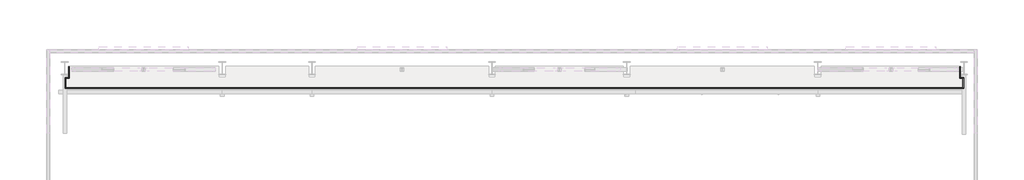
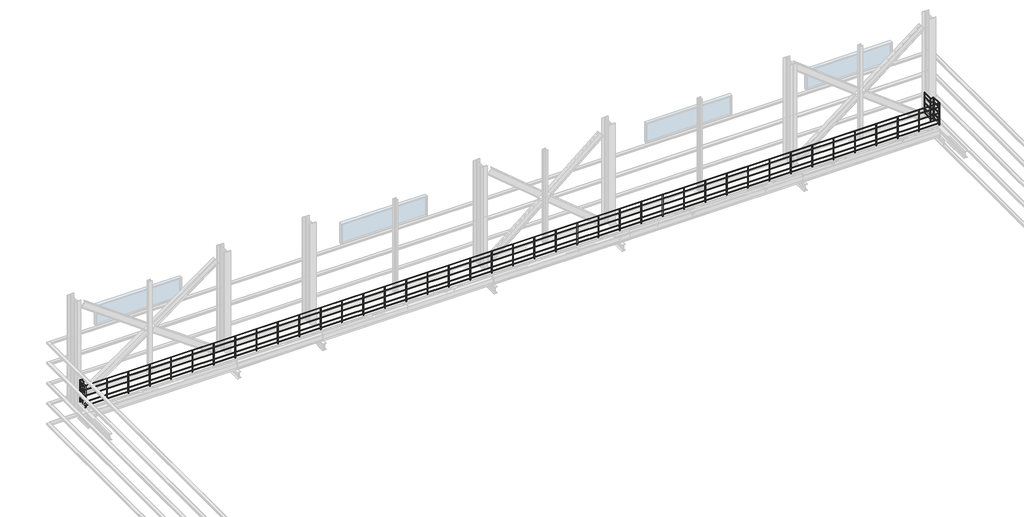
# One storey, part 4 of 4: 1 railing.
"""IFC4 building model written with IfcOpenShell, lengths in millimetres."""

import ifcopenshell
import ifcopenshell.guid

model = None  # the IFC model being written
_history = None  # IfcOwnerHistory: only IFC2X3 demands one
_inside = {}  # id of a spatial element -> (the spatial element, [elements in it])
_under = {}  # id of a project, library or spatial element -> (it, [spatial elements below it])
_declared = {}  # id of a project -> (the project, [libraries it declares])
_typed = {}  # id of a type object -> (the type object, [elements of that type])
_made_of = {}  # id of a material, layer set ... -> (it, [elements and type objects made of it])


def new_model(schema):
    """Start an empty IFC model of exactly this schema.

    Asked for "IFC4X3", IfcOpenShell would pick the latest addendum, in which some entities
    have other attributes; the version numbers below select the first issue.
    IFC2X3 requires an IfcOwnerHistory on every rooted entity: one is made here for all.
    """
    global model, _history
    if schema == "IFC4X3":
        model = ifcopenshell.file(schema_version=(4, 3, 0, 0))
    else:
        model = ifcopenshell.file(schema=schema)
    _inside.clear()
    _under.clear()
    _declared.clear()
    _typed.clear()
    _made_of.clear()
    _history = None
    if model.schema == "IFC2X3":
        org = make("IfcOrganization", Name="unknown")
        user = make(
            "IfcPersonAndOrganization",
            ThePerson=make("IfcPerson", FamilyName="unknown"),
            TheOrganization=org,
        )
        app = make(
            "IfcApplication",
            ApplicationDeveloper=org,
            Version="unknown",
            ApplicationFullName="unknown",
            ApplicationIdentifier="unknown",
        )
        _history = make(
            "IfcOwnerHistory",
            OwningUser=user,
            OwningApplication=app,
            ChangeAction="ADDED",
            CreationDate=0,
        )
    return model


def make(cls, **values):
    """One entity of the class cls with the attributes given. An attribute that is None is left unset."""
    return model.create_entity(
        cls, **{name: value for name, value in values.items() if value is not None}
    )


def rooted(cls, **values):
    """An entity with a GlobalId (a new one), such as an element, a storey or a relation."""
    return make(cls, GlobalId=ifcopenshell.guid.new(), OwnerHistory=_history, **values)


def si_unit(unit_type, name, prefix=None):
    """IfcSIUnit, for example si_unit("LENGTHUNIT", "METRE", prefix="MILLI")."""
    return make("IfcSIUnit", UnitType=unit_type, Prefix=prefix, Name=name)


def assignment(units):
    """IfcUnitAssignment: the units of a project."""
    return None if units is None else make("IfcUnitAssignment", Units=units)


def point(xyz):
    """IfcCartesianPoint."""
    return None if xyz is None else make("IfcCartesianPoint", Coordinates=xyz)


def direction(xyz):
    """IfcDirection."""
    return None if xyz is None else make("IfcDirection", DirectionRatios=xyz)


def frame(location, z_axis=None, x_axis=None):
    """IfcAxis2Placement3D, a coordinate frame: its origin and axes. An axis left out is left unset."""
    return make(
        "IfcAxis2Placement3D",
        Location=point(location),
        Axis=direction(z_axis),
        RefDirection=direction(x_axis),
    )


def origin():
    """The frame at (0, 0, 0) with its axes left unset."""
    return frame((0.0, 0.0, 0.0))


def place(relative_to, where):
    """IfcLocalPlacement: puts the frame where relative to a parent placement (None: the world)."""
    return make(
        "IfcLocalPlacement", PlacementRelTo=relative_to, RelativePlacement=where
    )


def context(
    kind, dimensions, precision=None, world=None, true_north=None, identifier=None
):
    """IfcGeometricRepresentationContext, for example the 3D "Model" context."""
    return make(
        "IfcGeometricRepresentationContext",
        ContextIdentifier=identifier,
        ContextType=kind,
        CoordinateSpaceDimension=dimensions,
        Precision=precision,
        WorldCoordinateSystem=world,
        TrueNorth=true_north,
    )


def project(units=None, contexts=None):
    """IfcProject with its units and contexts."""
    return rooted(
        "IfcProject",
        Name="project",
        RepresentationContexts=contexts,
        UnitsInContext=assignment(units),
    )


def spatial(cls, under=None, at=None, **own):
    """A site, building, storey or space (cls), placed at a placement, below another one or the project."""
    s = rooted(cls, ObjectPlacement=at, **own)
    if under is not None:
        _under.setdefault(under.id(), (under, []))[1].append(s)
    return s


def polyline(points):
    """IfcPolyline through the points."""
    return make("IfcPolyline", Points=[point(p) for p in points])


def circle_curve(where, radius):
    """IfcCircle in the frame where."""
    return make("IfcCircle", Position=where, Radius=radius)


def ellipse_curve(where, semi_axis1, semi_axis2):
    """IfcEllipse in the frame where."""
    return make(
        "IfcEllipse", Position=where, SemiAxis1=semi_axis1, SemiAxis2=semi_axis2
    )


def outline(outer, holes=None, kind="AREA"):
    """IfcArbitraryClosedProfileDef: a profile drawn as a closed curve; with holes, ...WithVoids."""
    if holes is None:
        return make("IfcArbitraryClosedProfileDef", ProfileType=kind, OuterCurve=outer)
    return make(
        "IfcArbitraryProfileDefWithVoids",
        ProfileType=kind,
        OuterCurve=outer,
        InnerCurves=holes,
    )


def extrude(swept, where, along, depth):
    """IfcExtrudedAreaSolid: the profile swept, set in the frame where, extruded along a direction by depth."""
    return make(
        "IfcExtrudedAreaSolid",
        SweptArea=swept,
        Position=where,
        ExtrudedDirection=direction(along),
        Depth=depth,
    )


def shape(context_of_items, identifier, shape_type, items):
    """IfcShapeRepresentation: the items that make up one representation, for example the "Body"."""
    return make(
        "IfcShapeRepresentation",
        ContextOfItems=context_of_items,
        RepresentationIdentifier=identifier,
        RepresentationType=shape_type,
        Items=items,
    )


def made_of(thing, what):
    """Note that an element or type object is made of a material, layer set ...; save() writes the relation."""
    if what is not None:
        _made_of.setdefault(what.id(), (what, []))[1].append(thing)
    return thing


def element(
    cls,
    number,
    at=None,
    inside=None,
    cuts=None,
    type_object=None,
    material=None,
    context=None,
    identifier="Body",
    shape_type=None,
    held_by="IfcProductDefinitionShape",
    body=None,
    shapes=None,
    **own,
):
    """One element of the class cls, such as IfcWall. Its Tag is "e" and its number.

    at: its placement. inside: the storey or other place that contains it. cuts: it is an
    opening in that element (IfcRelVoidsElement). A single representation is given by context,
    identifier, shape_type and body (its items); several are given by shapes. held_by: the class
    of the entity that holds the representations. save() writes the other relations.
    """
    e = rooted(cls, Tag="e%d" % number, ObjectPlacement=at, **own)
    if body is not None:
        shapes = [shape(context, identifier, shape_type, body)]
    if shapes is not None:
        e.Representation = make(held_by, Representations=shapes)
    if inside is not None:
        _inside.setdefault(inside.id(), (inside, []))[1].append(e)
    if cuts is not None:
        rooted(
            "IfcRelVoidsElement", RelatingBuildingElement=cuts, RelatedOpeningElement=e
        )
    if type_object is not None:
        _typed.setdefault(type_object.id(), (type_object, []))[1].append(e)
    return made_of(e, material)


def aggregate(whole, parts):
    """IfcRelAggregates: a whole, such as a stair, and the parts it consists of."""
    return rooted("IfcRelAggregates", RelatingObject=whole, RelatedObjects=parts)


def save(model, path):
    """Write the relations noted so far, then the file.

    IfcRelAggregates (storeys below a building ...), IfcRelContainedInSpatialStructure (elements
    in a storey), IfcRelDefinesByType, IfcRelAssociatesMaterial and IfcRelDeclares: one each for
    every whole, place, type object, material and project.
    """
    for whole, parts in _under.values():
        aggregate(whole, parts)
    for where, things in _inside.values():
        rooted(
            "IfcRelContainedInSpatialStructure",
            RelatedElements=things,
            RelatingStructure=where,
        )
    for kind, things in _typed.values():
        rooted("IfcRelDefinesByType", RelatedObjects=things, RelatingType=kind)
    for what, things in _made_of.values():
        rooted("IfcRelAssociatesMaterial", RelatedObjects=things, RelatingMaterial=what)
    for by, libraries in _declared.values():
        rooted("IfcRelDeclares", RelatingContext=by, RelatedDefinitions=libraries)
    model.write(path)


def plane_surface(at):
    """IfcPlane: the flat surface through the origin of the frame at, square to its z axis."""
    return make("IfcPlane", Position=at)


def cylinder_surface(at, radius):
    """IfcCylindricalSurface: all points at the distance radius from the z axis of the frame at."""
    return make("IfcCylindricalSurface", Position=at, Radius=radius)


def advanced_brep(points, edges, surfaces, faces):
    """IfcAdvancedBrep: a solid bounded by faces that lie on surfaces and meet in shared edges.

    An edge is (start, end): straight between two places in points (the first is 0);
    or (start, end, curve); or (start, end, curve, False) where it runs against its curve.
    A face is (place in surfaces, loops), or (place, loops, False) where it looks against
    its surface's normal. A loop lists edges by number (the first is 1), with a minus sign
    where the edge is run from its end to its start. The first loop is the outer one.
    """
    corners = [point(p) for p in points]
    vertices = [make("IfcVertexPoint", VertexGeometry=c) for c in corners]
    made = []
    for start, end, *more in edges:
        made.append(
            make(
                "IfcEdgeCurve",
                EdgeStart=vertices[start],
                EdgeEnd=vertices[end],
                EdgeGeometry=more[0] if more else make("IfcPolyline", Points=[corners[start], corners[end]]),
                SameSense=more[1] if len(more) > 1 else True,
            )
        )
    hull = []
    for where, loops, *sense in faces:
        bounds = []
        for j, loop in enumerate(loops):
            ring = [make("IfcOrientedEdge", EdgeElement=made[abs(k) - 1], Orientation=k > 0) for k in loop]
            bounds.append(
                make(
                    "IfcFaceOuterBound" if j == 0 else "IfcFaceBound",
                    Bound=make("IfcEdgeLoop", EdgeList=ring),
                    Orientation=True,
                )
            )
        hull.append(make("IfcAdvancedFace", Bounds=bounds, FaceSurface=surfaces[where], SameSense=sense[0] if sense else True))
    return make("IfcAdvancedBrep", Outer=make("IfcClosedShell", CfsFaces=hull))


model = new_model("IFC4")

# Units and contexts
model_context = context("Model", 3, world=origin())
ifc_project = project(units=[si_unit("LENGTHUNIT", "METRE", prefix="MILLI")], contexts=[model_context])

# Site, building, storey
site = spatial("IfcSite", under=ifc_project)
building = spatial("IfcBuilding", under=site)
storey = spatial("IfcBuildingStorey", under=building, Name="T.O.CRANE GIR.", Elevation=12299.9720055)

# Railing
placement = place(None, origin())
element("IfcRailing", 1, ObjectType="RA101_1100mm", at=placement, inside=storey, context=model_context, shape_type="SolidModel", body=[
    advanced_brep(
    [(165.0, 39119.5208589, 13466.9720055), (195.0, 39119.5208589, 13466.9720055), (165.0, 38634.5208589, 13466.9720055), (195.0, 38604.5208589, 13466.9720055), (15.0, 38634.5208589, 13466.9720055), (45.0, 38604.5208589, 13466.9720055), (15.0, 38164.5208589, 13466.9720055), (45.0, 38194.5208589, 13466.9720055), (39985.0, 38164.5208589, 13466.9720055), (39955.0, 38194.5208589, 13466.9720055), (39985.0, 38634.5208589, 13466.9720055), (39955.0, 38604.5208589, 13466.9720055), (39835.0, 38634.5208589, 13466.9720055), (39805.0, 38604.5208589, 13466.9720055), (39835.0, 39119.5208589, 13466.9720055), (39805.0, 39119.5208589, 13466.9720055)],
    [
        (0, 1, circle_curve(frame((180.0, 39119.5208589, 13466.9720055), z_axis=(0.0, 1.0, 0.0), x_axis=(1.0, 0.0, 0.0)), 15.0)),
        (1, 0, circle_curve(frame((180.0, 39119.5208589, 13466.9720055), z_axis=(0.0, 1.0, 0.0), x_axis=(1.0, 0.0, 0.0)), 15.0)),
        (0, 2),
        (2, 3, ellipse_curve(frame((180.0, 38619.5208589, 13466.9720055), z_axis=(0.707106781186548, 0.7071067811865469, 0.0), x_axis=(-0.7071067811865468, 0.7071067811865482, 0.0)), 21.2132034, 15.0)),
        (3, 1),
        (3, 2, ellipse_curve(frame((180.0, 38619.5208589, 13466.9720055), z_axis=(0.707106781186548, 0.7071067811865469, 0.0), x_axis=(-0.7071067811865468, 0.7071067811865482, 0.0)), 21.2132034, 15.0)),
        (2, 4),
        (4, 5, ellipse_curve(frame((30.0, 38619.5208589, 13466.9720055), z_axis=(0.707106781186548, 0.7071067811865469, 0.0), x_axis=(0.7071067811865472, -0.7071067811865479, 0.0)), 21.2132034, 15.0)),
        (5, 3),
        (5, 4, ellipse_curve(frame((30.0, 38619.5208589, 13466.9720055), z_axis=(0.707106781186548, 0.7071067811865469, 0.0), x_axis=(0.7071067811865472, -0.7071067811865479, 0.0)), 21.2132034, 15.0)),
        (4, 6),
        (6, 7, ellipse_curve(frame((30.0, 38179.5208589, 13466.9720055), z_axis=(-0.7071067811865459, 0.7071067811865491, 0.0), x_axis=(0.7071067811865491, 0.7071067811865458, 0.0)), 21.2132034, 15.0)),
        (7, 5),
        (7, 6, ellipse_curve(frame((30.0, 38179.5208589, 13466.9720055), z_axis=(-0.7071067811865459, 0.7071067811865491, 0.0), x_axis=(0.7071067811865491, 0.7071067811865458, 0.0)), 21.2132034, 15.0)),
        (6, 8),
        (8, 9, ellipse_curve(frame((39970.0, 38179.5208589, 13466.9720055), z_axis=(-0.7071067811865486, -0.7071067811865465, 0.0), x_axis=(-0.7071067811865465, 0.7071067811865486, 0.0)), 21.2132034, 15.0)),
        (9, 7),
        (9, 8, ellipse_curve(frame((39970.0, 38179.5208589, 13466.9720055), z_axis=(-0.7071067811865486, -0.7071067811865465, 0.0), x_axis=(-0.7071067811865465, 0.7071067811865486, 0.0)), 21.2132034, 15.0)),
        (8, 10),
        (10, 11, ellipse_curve(frame((39970.0, 38619.5208589, 13466.9720055), z_axis=(0.7071067811865476, -0.7071067811865474, 0.0), x_axis=(-0.7071067811865472, -0.7071067811865478, 0.0)), 21.2132034, 15.0)),
        (11, 9),
        (11, 10, ellipse_curve(frame((39970.0, 38619.5208589, 13466.9720055), z_axis=(0.7071067811865476, -0.7071067811865474, 0.0), x_axis=(-0.7071067811865472, -0.7071067811865478, 0.0)), 21.2132034, 15.0)),
        (10, 12),
        (12, 13, ellipse_curve(frame((39820.0, 38619.5208589, 13466.9720055), z_axis=(0.7071067811865476, -0.7071067811865474, 0.0), x_axis=(0.7071067811865475, 0.7071067811865475, 0.0)), 21.2132034, 15.0)),
        (13, 11),
        (13, 12, ellipse_curve(frame((39820.0, 38619.5208589, 13466.9720055), z_axis=(0.7071067811865476, -0.7071067811865474, 0.0), x_axis=(0.7071067811865475, 0.7071067811865475, 0.0)), 21.2132034, 15.0)),
        (14, 15, circle_curve(frame((39820.0, 39119.5208589, 13466.9720055), z_axis=(0.0, 1.0, 0.0), x_axis=(-1.0, 0.0, 0.0)), 15.0)),
        (15, 14, circle_curve(frame((39820.0, 39119.5208589, 13466.9720055), z_axis=(0.0, 1.0, 0.0), x_axis=(-1.0, 0.0, 0.0)), 15.0)),
        (12, 14),
        (15, 13),
    ],
    [
        plane_surface(frame((180.0, 39119.5208589, 13481.9720055), z_axis=(0.0, 1.0, 0.0), x_axis=(0.0, 0.0, -1.0))),
        cylinder_surface(frame((180.0, 39119.5208589, 13466.9720055), z_axis=(0.0, 1.0, 0.0), x_axis=(1.0, 0.0, 0.0)), 15.0),
        cylinder_surface(frame((180.0, 38619.5208589, 13466.9720055), z_axis=(1.0, 0.0, 0.0), x_axis=(0.0, -1.0, 0.0)), 15.0),
        cylinder_surface(frame((30.0, 38619.5208589, 13466.9720055), z_axis=(0.0, 1.0, 0.0), x_axis=(1.0, 0.0, 0.0)), 15.0),
        cylinder_surface(frame((30.0, 38179.5208589, 13466.9720055), z_axis=(-1.0, 0.0, 0.0), x_axis=(0.0, 1.0, 0.0)), 15.0),
        cylinder_surface(frame((39970.0, 38179.5208589, 13466.9720055), z_axis=(0.0, -1.0, 0.0), x_axis=(-1.0, 0.0, 0.0)), 15.0),
        cylinder_surface(frame((39970.0, 38619.5208589, 13466.9720055), z_axis=(1.0, 0.0, 0.0), x_axis=(0.0, -1.0, 0.0)), 15.0),
        plane_surface(frame((39820.0, 39119.5208589, 13481.9720055), z_axis=(0.0, 1.0, 0.0), x_axis=(0.0, 0.0, 1.0))),
        cylinder_surface(frame((39820.0, 38619.5208589, 13466.9720055), z_axis=(0.0, -1.0, 0.0), x_axis=(-1.0, 0.0, 0.0)), 15.0),
    ],
    [
        (0, [[1, 2]]),
        (1, [[-1, 3, 4, 5]]),
        (1, [[-2, -5, 6, -3]]),
        (2, [[-4, 7, 8, 9]]),
        (2, [[-6, -9, 10, -7]]),
        (3, [[-8, 11, 12, 13]]),
        (3, [[-10, -13, 14, -11]]),
        (4, [[-12, 15, 16, 17]]),
        (4, [[-14, -17, 18, -15]]),
        (5, [[-16, 19, 20, 21]]),
        (5, [[-18, -21, 22, -19]]),
        (6, [[-20, 23, 24, 25]]),
        (6, [[-22, -25, 26, -23]]),
        (7, [[27, 28]]),
        (8, [[-24, 29, -28, 30]]),
        (8, [[-26, -30, -27, -29]]),
    ],
),
    advanced_brep(
    [(15.0, 38634.5208589, 13266.9720055), (45.0, 38604.5208589, 13266.9720055), (45.0, 38194.5208589, 13266.9720055), (15.0, 38164.5208589, 13266.9720055), (39955.0, 38194.5208589, 13266.9720055), (39985.0, 38164.5208589, 13266.9720055), (39955.0, 38604.5208589, 13266.9720055), (39985.0, 38634.5208589, 13266.9720055), (39805.0, 38604.5208589, 13266.9720055), (39835.0, 38634.5208589, 13266.9720055), (39805.0, 39119.5208589, 13266.9720055), (39835.0, 39119.5208589, 13266.9720055), (195.0, 39119.5208589, 13266.9720055), (165.0, 39119.5208589, 13266.9720055), (195.0, 38604.5208589, 13266.9720055), (165.0, 38634.5208589, 13266.9720055)],
    [
        (0, 1, ellipse_curve(frame((30.0, 38619.5208589, 13266.9720055), z_axis=(-0.707106781186548, -0.7071067811865469, 0.0), x_axis=(-0.7071067811865467, 0.7071067811865482, 0.0)), 21.2132034, 15.0)),
        (1, 2),
        (2, 3, ellipse_curve(frame((30.0, 38179.5208589, 13266.9720055), z_axis=(-0.7071067811865459, 0.7071067811865491, 0.0), x_axis=(0.7071067811865491, 0.7071067811865458, 0.0)), 21.2132034, 15.0)),
        (3, 0),
        (1, 0, ellipse_curve(frame((30.0, 38619.5208589, 13266.9720055), z_axis=(-0.707106781186548, -0.7071067811865469, 0.0), x_axis=(-0.7071067811865467, 0.7071067811865482, 0.0)), 21.2132034, 15.0)),
        (3, 2, ellipse_curve(frame((30.0, 38179.5208589, 13266.9720055), z_axis=(-0.7071067811865459, 0.7071067811865491, 0.0), x_axis=(0.7071067811865491, 0.7071067811865458, 0.0)), 21.2132034, 15.0)),
        (2, 4),
        (4, 5, ellipse_curve(frame((39970.0, 38179.5208589, 13266.9720055), z_axis=(-0.7071067811865486, -0.7071067811865465, 0.0), x_axis=(-0.7071067811865465, 0.7071067811865486, 0.0)), 21.2132034, 15.0)),
        (5, 3),
        (5, 4, ellipse_curve(frame((39970.0, 38179.5208589, 13266.9720055), z_axis=(-0.7071067811865486, -0.7071067811865465, 0.0), x_axis=(-0.7071067811865465, 0.7071067811865486, 0.0)), 21.2132034, 15.0)),
        (4, 6),
        (6, 7, ellipse_curve(frame((39970.0, 38619.5208589, 13266.9720055), z_axis=(0.7071067811865476, -0.7071067811865474, 0.0), x_axis=(-0.7071067811865472, -0.7071067811865478, 0.0)), 21.2132034, 15.0)),
        (7, 5),
        (7, 6, ellipse_curve(frame((39970.0, 38619.5208589, 13266.9720055), z_axis=(0.7071067811865476, -0.7071067811865474, 0.0), x_axis=(-0.7071067811865472, -0.7071067811865478, 0.0)), 21.2132034, 15.0)),
        (6, 8),
        (8, 9, ellipse_curve(frame((39820.0, 38619.5208589, 13266.9720055), z_axis=(0.7071067811865476, -0.7071067811865474, 0.0), x_axis=(0.7071067811865475, 0.7071067811865475, 0.0)), 21.2132034, 15.0)),
        (9, 7),
        (9, 8, ellipse_curve(frame((39820.0, 38619.5208589, 13266.9720055), z_axis=(0.7071067811865476, -0.7071067811865474, 0.0), x_axis=(0.7071067811865475, 0.7071067811865475, 0.0)), 21.2132034, 15.0)),
        (10, 11, circle_curve(frame((39820.0, 39119.5208589, 13266.9720055), z_axis=(0.0, 1.0, 0.0), x_axis=(1.0, 0.0, 0.0)), 15.0)),
        (11, 10, circle_curve(frame((39820.0, 39119.5208589, 13266.9720055), z_axis=(0.0, 1.0, 0.0), x_axis=(1.0, 0.0, 0.0)), 15.0)),
        (8, 10),
        (11, 9),
        (12, 13, circle_curve(frame((180.0, 39119.5208589, 13266.9720055), z_axis=(0.0, 1.0, 0.0), x_axis=(-1.0, 0.0, 0.0)), 15.0)),
        (13, 12, circle_curve(frame((180.0, 39119.5208589, 13266.9720055), z_axis=(0.0, 1.0, 0.0), x_axis=(-1.0, 0.0, 0.0)), 15.0)),
        (12, 14),
        (14, 15, ellipse_curve(frame((180.0, 38619.5208589, 13266.9720055), z_axis=(0.707106781186548, 0.7071067811865469, 0.0), x_axis=(-0.7071067811865468, 0.7071067811865482, 0.0)), 21.2132034, 15.0)),
        (15, 13),
        (15, 14, ellipse_curve(frame((180.0, 38619.5208589, 13266.9720055), z_axis=(0.707106781186548, 0.7071067811865469, 0.0), x_axis=(-0.7071067811865468, 0.7071067811865482, 0.0)), 21.2132034, 15.0)),
        (14, 1),
        (0, 15),
    ],
    [
        cylinder_surface(frame((30.0, 38619.5208589, 13266.9720055), z_axis=(0.0, 1.0, 0.0), x_axis=(-1.0, 0.0, 0.0)), 15.0),
        cylinder_surface(frame((30.0, 38179.5208589, 13266.9720055), z_axis=(-1.0, 0.0, 0.0), x_axis=(0.0, -1.0, 0.0)), 15.0),
        cylinder_surface(frame((39970.0, 38179.5208589, 13266.9720055), z_axis=(0.0, -1.0, 0.0), x_axis=(1.0, 0.0, 0.0)), 15.0),
        cylinder_surface(frame((39970.0, 38619.5208589, 13266.9720055), z_axis=(1.0, 0.0, 0.0), x_axis=(0.0, 1.0, 0.0)), 15.0),
        plane_surface(frame((39820.0, 39119.5208589, 13281.9720055), z_axis=(0.0, 1.0, 0.0), x_axis=(0.0, 0.0, 1.0))),
        cylinder_surface(frame((39820.0, 38619.5208589, 13266.9720055), z_axis=(0.0, -1.0, 0.0), x_axis=(1.0, 0.0, 0.0)), 15.0),
        plane_surface(frame((180.0, 39119.5208589, 13281.9720055), z_axis=(0.0, 1.0, 0.0), x_axis=(0.0, 0.0, -1.0))),
        cylinder_surface(frame((180.0, 39119.5208589, 13266.9720055), z_axis=(0.0, 1.0, 0.0), x_axis=(-1.0, 0.0, 0.0)), 15.0),
        cylinder_surface(frame((180.0, 38619.5208589, 13266.9720055), z_axis=(1.0, 0.0, 0.0), x_axis=(0.0, 1.0, 0.0)), 15.0),
    ],
    [
        (0, [[1, 2, 3, 4]]),
        (0, [[5, -4, 6, -2]]),
        (1, [[-3, 7, 8, 9]]),
        (1, [[-6, -9, 10, -7]]),
        (2, [[-8, 11, 12, 13]]),
        (2, [[-10, -13, 14, -11]]),
        (3, [[-12, 15, 16, 17]]),
        (3, [[-14, -17, 18, -15]]),
        (4, [[19, 20]]),
        (5, [[-16, 21, -20, 22]]),
        (5, [[-18, -22, -19, -21]]),
        (6, [[23, 24]]),
        (7, [[-23, 25, 26, 27]]),
        (7, [[-24, -27, 28, -25]]),
        (8, [[-26, 29, -1, 30]]),
        (8, [[-28, -30, -5, -29]]),
    ],
),
    advanced_brep(
    [(15.0, 38634.5208589, 12966.9720055), (45.0, 38604.5208589, 12966.9720055), (45.0, 38194.5208589, 12966.9720055), (15.0, 38164.5208589, 12966.9720055), (39955.0, 38194.5208589, 12966.9720055), (39985.0, 38164.5208589, 12966.9720055), (39955.0, 38604.5208589, 12966.9720055), (39985.0, 38634.5208589, 12966.9720055), (39805.0, 38604.5208589, 12966.9720055), (39835.0, 38634.5208589, 12966.9720055), (39805.0, 39119.5208589, 12966.9720055), (39835.0, 39119.5208589, 12966.9720055), (195.0, 39119.5208589, 12966.9720055), (165.0, 39119.5208589, 12966.9720055), (195.0, 38604.5208589, 12966.9720055), (165.0, 38634.5208589, 12966.9720055)],
    [
        (0, 1, ellipse_curve(frame((30.0, 38619.5208589, 12966.9720055), z_axis=(-0.707106781186548, -0.7071067811865469, 0.0), x_axis=(-0.7071067811865467, 0.7071067811865482, 0.0)), 21.2132034, 15.0)),
        (1, 2),
        (2, 3, ellipse_curve(frame((30.0, 38179.5208589, 12966.9720055), z_axis=(-0.7071067811865459, 0.7071067811865491, 0.0), x_axis=(0.7071067811865491, 0.7071067811865458, 0.0)), 21.2132034, 15.0)),
        (3, 0),
        (1, 0, ellipse_curve(frame((30.0, 38619.5208589, 12966.9720055), z_axis=(-0.707106781186548, -0.7071067811865469, 0.0), x_axis=(-0.7071067811865467, 0.7071067811865482, 0.0)), 21.2132034, 15.0)),
        (3, 2, ellipse_curve(frame((30.0, 38179.5208589, 12966.9720055), z_axis=(-0.7071067811865459, 0.7071067811865491, 0.0), x_axis=(0.7071067811865491, 0.7071067811865458, 0.0)), 21.2132034, 15.0)),
        (2, 4),
        (4, 5, ellipse_curve(frame((39970.0, 38179.5208589, 12966.9720055), z_axis=(-0.7071067811865486, -0.7071067811865465, 0.0), x_axis=(-0.7071067811865465, 0.7071067811865486, 0.0)), 21.2132034, 15.0)),
        (5, 3),
        (5, 4, ellipse_curve(frame((39970.0, 38179.5208589, 12966.9720055), z_axis=(-0.7071067811865486, -0.7071067811865465, 0.0), x_axis=(-0.7071067811865465, 0.7071067811865486, 0.0)), 21.2132034, 15.0)),
        (4, 6),
        (6, 7, ellipse_curve(frame((39970.0, 38619.5208589, 12966.9720055), z_axis=(0.7071067811865476, -0.7071067811865474, 0.0), x_axis=(-0.7071067811865472, -0.7071067811865478, 0.0)), 21.2132034, 15.0)),
        (7, 5),
        (7, 6, ellipse_curve(frame((39970.0, 38619.5208589, 12966.9720055), z_axis=(0.7071067811865476, -0.7071067811865474, 0.0), x_axis=(-0.7071067811865472, -0.7071067811865478, 0.0)), 21.2132034, 15.0)),
        (6, 8),
        (8, 9, ellipse_curve(frame((39820.0, 38619.5208589, 12966.9720055), z_axis=(0.7071067811865476, -0.7071067811865474, 0.0), x_axis=(0.7071067811865475, 0.7071067811865475, 0.0)), 21.2132034, 15.0)),
        (9, 7),
        (9, 8, ellipse_curve(frame((39820.0, 38619.5208589, 12966.9720055), z_axis=(0.7071067811865476, -0.7071067811865474, 0.0), x_axis=(0.7071067811865475, 0.7071067811865475, 0.0)), 21.2132034, 15.0)),
        (10, 11, circle_curve(frame((39820.0, 39119.5208589, 12966.9720055), z_axis=(0.0, 1.0, 0.0), x_axis=(1.0, 0.0, 0.0)), 15.0)),
        (11, 10, circle_curve(frame((39820.0, 39119.5208589, 12966.9720055), z_axis=(0.0, 1.0, 0.0), x_axis=(1.0, 0.0, 0.0)), 15.0)),
        (8, 10),
        (11, 9),
        (12, 13, circle_curve(frame((180.0, 39119.5208589, 12966.9720055), z_axis=(0.0, 1.0, 0.0), x_axis=(-1.0, 0.0, 0.0)), 15.0)),
        (13, 12, circle_curve(frame((180.0, 39119.5208589, 12966.9720055), z_axis=(0.0, 1.0, 0.0), x_axis=(-1.0, 0.0, 0.0)), 15.0)),
        (12, 14),
        (14, 15, ellipse_curve(frame((180.0, 38619.5208589, 12966.9720055), z_axis=(0.707106781186548, 0.7071067811865469, 0.0), x_axis=(-0.7071067811865468, 0.7071067811865482, 0.0)), 21.2132034, 15.0)),
        (15, 13),
        (15, 14, ellipse_curve(frame((180.0, 38619.5208589, 12966.9720055), z_axis=(0.707106781186548, 0.7071067811865469, 0.0), x_axis=(-0.7071067811865468, 0.7071067811865482, 0.0)), 21.2132034, 15.0)),
        (14, 1),
        (0, 15),
    ],
    [
        cylinder_surface(frame((30.0, 38619.5208589, 12966.9720055), z_axis=(0.0, 1.0, 0.0), x_axis=(-1.0, 0.0, 0.0)), 15.0),
        cylinder_surface(frame((30.0, 38179.5208589, 12966.9720055), z_axis=(-1.0, 0.0, 0.0), x_axis=(0.0, -1.0, 0.0)), 15.0),
        cylinder_surface(frame((39970.0, 38179.5208589, 12966.9720055), z_axis=(0.0, -1.0, 0.0), x_axis=(1.0, 0.0, 0.0)), 15.0),
        cylinder_surface(frame((39970.0, 38619.5208589, 12966.9720055), z_axis=(1.0, 0.0, 0.0), x_axis=(0.0, 1.0, 0.0)), 15.0),
        plane_surface(frame((39820.0, 39119.5208589, 12981.9720055), z_axis=(0.0, 1.0, 0.0), x_axis=(0.0, 0.0, 1.0))),
        cylinder_surface(frame((39820.0, 38619.5208589, 12966.9720055), z_axis=(0.0, -1.0, 0.0), x_axis=(1.0, 0.0, 0.0)), 15.0),
        plane_surface(frame((180.0, 39119.5208589, 12981.9720055), z_axis=(0.0, 1.0, 0.0), x_axis=(0.0, 0.0, -1.0))),
        cylinder_surface(frame((180.0, 39119.5208589, 12966.9720055), z_axis=(0.0, 1.0, 0.0), x_axis=(-1.0, 0.0, 0.0)), 15.0),
        cylinder_surface(frame((180.0, 38619.5208589, 12966.9720055), z_axis=(1.0, 0.0, 0.0), x_axis=(0.0, 1.0, 0.0)), 15.0),
    ],
    [
        (0, [[1, 2, 3, 4]]),
        (0, [[5, -4, 6, -2]]),
        (1, [[-3, 7, 8, 9]]),
        (1, [[-6, -9, 10, -7]]),
        (2, [[-8, 11, 12, 13]]),
        (2, [[-10, -13, 14, -11]]),
        (3, [[-12, 15, 16, 17]]),
        (3, [[-14, -17, 18, -15]]),
        (4, [[19, 20]]),
        (5, [[-16, 21, -20, 22]]),
        (5, [[-18, -22, -19, -21]]),
        (6, [[23, 24]]),
        (7, [[-23, 25, 26, 27]]),
        (7, [[-24, -27, 28, -25]]),
        (8, [[-26, 29, -1, 30]]),
        (8, [[-28, -30, -5, -29]]),
    ],
),
    advanced_brep(
    [(195.0, 39119.5208589, 12666.9720055), (165.0, 39119.5208589, 12666.9720055), (195.0, 38604.5208589, 12666.9720055), (165.0, 38634.5208589, 12666.9720055), (45.0, 38604.5208589, 12666.9720055), (15.0, 38634.5208589, 12666.9720055), (45.0, 38194.5208589, 12666.9720055), (15.0, 38164.5208589, 12666.9720055), (39955.0, 38194.5208589, 12666.9720055), (39985.0, 38164.5208589, 12666.9720055), (39955.0, 38604.5208589, 12666.9720055), (39985.0, 38634.5208589, 12666.9720055), (39805.0, 38604.5208589, 12666.9720055), (39835.0, 38634.5208589, 12666.9720055), (39805.0, 39119.5208589, 12666.9720055), (39835.0, 39119.5208589, 12666.9720055)],
    [
        (0, 1, circle_curve(frame((180.0, 39119.5208589, 12666.9720055), z_axis=(0.0, 1.0, 0.0), x_axis=(-1.0, 0.0, 0.0)), 15.0)),
        (1, 0, circle_curve(frame((180.0, 39119.5208589, 12666.9720055), z_axis=(0.0, 1.0, 0.0), x_axis=(-1.0, 0.0, 0.0)), 15.0)),
        (0, 2),
        (2, 3, ellipse_curve(frame((180.0, 38619.5208589, 12666.9720055), z_axis=(0.707106781186548, 0.7071067811865469, 0.0), x_axis=(-0.7071067811865468, 0.7071067811865482, 0.0)), 21.2132034, 15.0)),
        (3, 1),
        (3, 2, ellipse_curve(frame((180.0, 38619.5208589, 12666.9720055), z_axis=(0.707106781186548, 0.7071067811865469, 0.0), x_axis=(-0.7071067811865468, 0.7071067811865482, 0.0)), 21.2132034, 15.0)),
        (2, 4),
        (4, 5, ellipse_curve(frame((30.0, 38619.5208589, 12666.9720055), z_axis=(0.707106781186548, 0.7071067811865469, 0.0), x_axis=(0.7071067811865472, -0.7071067811865479, 0.0)), 21.2132034, 15.0)),
        (5, 3),
        (5, 4, ellipse_curve(frame((30.0, 38619.5208589, 12666.9720055), z_axis=(0.707106781186548, 0.7071067811865469, 0.0), x_axis=(0.7071067811865472, -0.7071067811865479, 0.0)), 21.2132034, 15.0)),
        (4, 6),
        (6, 7, ellipse_curve(frame((30.0, 38179.5208589, 12666.9720055), z_axis=(-0.7071067811865459, 0.7071067811865491, 0.0), x_axis=(0.7071067811865491, 0.7071067811865458, 0.0)), 21.2132034, 15.0)),
        (7, 5),
        (7, 6, ellipse_curve(frame((30.0, 38179.5208589, 12666.9720055), z_axis=(-0.7071067811865459, 0.7071067811865491, 0.0), x_axis=(0.7071067811865491, 0.7071067811865458, 0.0)), 21.2132034, 15.0)),
        (6, 8),
        (8, 9, ellipse_curve(frame((39970.0, 38179.5208589, 12666.9720055), z_axis=(-0.7071067811865486, -0.7071067811865465, 0.0), x_axis=(-0.7071067811865465, 0.7071067811865486, 0.0)), 21.2132034, 15.0)),
        (9, 7),
        (9, 8, ellipse_curve(frame((39970.0, 38179.5208589, 12666.9720055), z_axis=(-0.7071067811865486, -0.7071067811865465, 0.0), x_axis=(-0.7071067811865465, 0.7071067811865486, 0.0)), 21.2132034, 15.0)),
        (8, 10),
        (10, 11, ellipse_curve(frame((39970.0, 38619.5208589, 12666.9720055), z_axis=(0.7071067811865476, -0.7071067811865474, 0.0), x_axis=(-0.7071067811865472, -0.7071067811865478, 0.0)), 21.2132034, 15.0)),
        (11, 9),
        (11, 10, ellipse_curve(frame((39970.0, 38619.5208589, 12666.9720055), z_axis=(0.7071067811865476, -0.7071067811865474, 0.0), x_axis=(-0.7071067811865472, -0.7071067811865478, 0.0)), 21.2132034, 15.0)),
        (10, 12),
        (12, 13, ellipse_curve(frame((39820.0, 38619.5208589, 12666.9720055), z_axis=(0.7071067811865476, -0.7071067811865474, 0.0), x_axis=(0.7071067811865475, 0.7071067811865475, 0.0)), 21.2132034, 15.0)),
        (13, 11),
        (13, 12, ellipse_curve(frame((39820.0, 38619.5208589, 12666.9720055), z_axis=(0.7071067811865476, -0.7071067811865474, 0.0), x_axis=(0.7071067811865475, 0.7071067811865475, 0.0)), 21.2132034, 15.0)),
        (14, 15, circle_curve(frame((39820.0, 39119.5208589, 12666.9720055), z_axis=(0.0, 1.0, 0.0), x_axis=(1.0, 0.0, 0.0)), 15.0)),
        (15, 14, circle_curve(frame((39820.0, 39119.5208589, 12666.9720055), z_axis=(0.0, 1.0, 0.0), x_axis=(1.0, 0.0, 0.0)), 15.0)),
        (12, 14),
        (15, 13),
    ],
    [
        plane_surface(frame((180.0, 39119.5208589, 12681.9720055), z_axis=(0.0, 1.0, 0.0), x_axis=(0.0, 0.0, -1.0))),
        cylinder_surface(frame((180.0, 39119.5208589, 12666.9720055), z_axis=(0.0, 1.0, 0.0), x_axis=(-1.0, 0.0, 0.0)), 15.0),
        cylinder_surface(frame((180.0, 38619.5208589, 12666.9720055), z_axis=(1.0, 0.0, 0.0), x_axis=(0.0, 1.0, 0.0)), 15.0),
        cylinder_surface(frame((30.0, 38619.5208589, 12666.9720055), z_axis=(0.0, 1.0, 0.0), x_axis=(-1.0, 0.0, 0.0)), 15.0),
        cylinder_surface(frame((30.0, 38179.5208589, 12666.9720055), z_axis=(-1.0, 0.0, 0.0), x_axis=(0.0, -1.0, 0.0)), 15.0),
        cylinder_surface(frame((39970.0, 38179.5208589, 12666.9720055), z_axis=(0.0, -1.0, 0.0), x_axis=(1.0, 0.0, 0.0)), 15.0),
        cylinder_surface(frame((39970.0, 38619.5208589, 12666.9720055), z_axis=(1.0, 0.0, 0.0), x_axis=(0.0, 1.0, 0.0)), 15.0),
        plane_surface(frame((39820.0, 39119.5208589, 12681.9720055), z_axis=(0.0, 1.0, 0.0), x_axis=(0.0, 0.0, 1.0))),
        cylinder_surface(frame((39820.0, 38619.5208589, 12666.9720055), z_axis=(0.0, -1.0, 0.0), x_axis=(1.0, 0.0, 0.0)), 15.0),
    ],
    [
        (0, [[1, 2]]),
        (1, [[-1, 3, 4, 5]]),
        (1, [[-2, -5, 6, -3]]),
        (2, [[-4, 7, 8, 9]]),
        (2, [[-6, -9, 10, -7]]),
        (3, [[-8, 11, 12, 13]]),
        (3, [[-10, -13, 14, -11]]),
        (4, [[-12, 15, 16, 17]]),
        (4, [[-14, -17, 18, -15]]),
        (5, [[-16, 19, 20, 21]]),
        (5, [[-18, -21, 22, -19]]),
        (6, [[-20, 23, 24, 25]]),
        (6, [[-22, -25, 26, -23]]),
        (7, [[27, 28]]),
        (8, [[-24, 29, -28, 30]]),
        (8, [[-26, -30, -27, -29]]),
    ],
),
    advanced_brep(
    [(195.0, 39119.5208589, 12466.9720055), (165.0, 39119.5208589, 12466.9720055), (195.0, 38604.5208589, 12466.9720055), (165.0, 38634.5208589, 12466.9720055), (45.0, 38604.5208589, 12466.9720055), (15.0, 38634.5208589, 12466.9720055), (45.0, 38194.5208589, 12466.9720055), (15.0, 38164.5208589, 12466.9720055), (39955.0, 38194.5208589, 12466.9720055), (39985.0, 38164.5208589, 12466.9720055), (39955.0, 38604.5208589, 12466.9720055), (39985.0, 38634.5208589, 12466.9720055), (39805.0, 38604.5208589, 12466.9720055), (39835.0, 38634.5208589, 12466.9720055), (39805.0, 39119.5208589, 12466.9720055), (39835.0, 39119.5208589, 12466.9720055)],
    [
        (0, 1, circle_curve(frame((180.0, 39119.5208589, 12466.9720055), z_axis=(0.0, 1.0, 0.0), x_axis=(-1.0, 0.0, 0.0)), 15.0)),
        (1, 0, circle_curve(frame((180.0, 39119.5208589, 12466.9720055), z_axis=(0.0, 1.0, 0.0), x_axis=(-1.0, 0.0, 0.0)), 15.0)),
        (0, 2),
        (2, 3, ellipse_curve(frame((180.0, 38619.5208589, 12466.9720055), z_axis=(0.707106781186548, 0.7071067811865469, 0.0), x_axis=(-0.7071067811865468, 0.7071067811865482, 0.0)), 21.2132034, 15.0)),
        (3, 1),
        (3, 2, ellipse_curve(frame((180.0, 38619.5208589, 12466.9720055), z_axis=(0.707106781186548, 0.7071067811865469, 0.0), x_axis=(-0.7071067811865468, 0.7071067811865482, 0.0)), 21.2132034, 15.0)),
        (2, 4),
        (4, 5, ellipse_curve(frame((30.0, 38619.5208589, 12466.9720055), z_axis=(0.707106781186548, 0.7071067811865469, 0.0), x_axis=(0.7071067811865472, -0.7071067811865479, 0.0)), 21.2132034, 15.0)),
        (5, 3),
        (5, 4, ellipse_curve(frame((30.0, 38619.5208589, 12466.9720055), z_axis=(0.707106781186548, 0.7071067811865469, 0.0), x_axis=(0.7071067811865472, -0.7071067811865479, 0.0)), 21.2132034, 15.0)),
        (4, 6),
        (6, 7, ellipse_curve(frame((30.0, 38179.5208589, 12466.9720055), z_axis=(-0.7071067811865459, 0.7071067811865491, 0.0), x_axis=(0.7071067811865491, 0.7071067811865458, 0.0)), 21.2132034, 15.0)),
        (7, 5),
        (7, 6, ellipse_curve(frame((30.0, 38179.5208589, 12466.9720055), z_axis=(-0.7071067811865459, 0.7071067811865491, 0.0), x_axis=(0.7071067811865491, 0.7071067811865458, 0.0)), 21.2132034, 15.0)),
        (6, 8),
        (8, 9, ellipse_curve(frame((39970.0, 38179.5208589, 12466.9720055), z_axis=(-0.7071067811865486, -0.7071067811865465, 0.0), x_axis=(-0.7071067811865465, 0.7071067811865486, 0.0)), 21.2132034, 15.0)),
        (9, 7),
        (9, 8, ellipse_curve(frame((39970.0, 38179.5208589, 12466.9720055), z_axis=(-0.7071067811865486, -0.7071067811865465, 0.0), x_axis=(-0.7071067811865465, 0.7071067811865486, 0.0)), 21.2132034, 15.0)),
        (8, 10),
        (10, 11, ellipse_curve(frame((39970.0, 38619.5208589, 12466.9720055), z_axis=(0.7071067811865476, -0.7071067811865474, 0.0), x_axis=(-0.7071067811865472, -0.7071067811865478, 0.0)), 21.2132034, 15.0)),
        (11, 9),
        (11, 10, ellipse_curve(frame((39970.0, 38619.5208589, 12466.9720055), z_axis=(0.7071067811865476, -0.7071067811865474, 0.0), x_axis=(-0.7071067811865472, -0.7071067811865478, 0.0)), 21.2132034, 15.0)),
        (10, 12),
        (12, 13, ellipse_curve(frame((39820.0, 38619.5208589, 12466.9720055), z_axis=(0.7071067811865476, -0.7071067811865474, 0.0), x_axis=(0.7071067811865475, 0.7071067811865475, 0.0)), 21.2132034, 15.0)),
        (13, 11),
        (13, 12, ellipse_curve(frame((39820.0, 38619.5208589, 12466.9720055), z_axis=(0.7071067811865476, -0.7071067811865474, 0.0), x_axis=(0.7071067811865475, 0.7071067811865475, 0.0)), 21.2132034, 15.0)),
        (14, 15, circle_curve(frame((39820.0, 39119.5208589, 12466.9720055), z_axis=(0.0, 1.0, 0.0), x_axis=(1.0, 0.0, 0.0)), 15.0)),
        (15, 14, circle_curve(frame((39820.0, 39119.5208589, 12466.9720055), z_axis=(0.0, 1.0, 0.0), x_axis=(1.0, 0.0, 0.0)), 15.0)),
        (12, 14),
        (15, 13),
    ],
    [
        plane_surface(frame((180.0, 39119.5208589, 12481.9720055), z_axis=(0.0, 1.0, 0.0), x_axis=(0.0, 0.0, -1.0))),
        cylinder_surface(frame((180.0, 39119.5208589, 12466.9720055), z_axis=(0.0, 1.0, 0.0), x_axis=(-1.0, 0.0, 0.0)), 15.0),
        cylinder_surface(frame((180.0, 38619.5208589, 12466.9720055), z_axis=(1.0, 0.0, 0.0), x_axis=(0.0, 1.0, 0.0)), 15.0),
        cylinder_surface(frame((30.0, 38619.5208589, 12466.9720055), z_axis=(0.0, 1.0, 0.0), x_axis=(-1.0, 0.0, 0.0)), 15.0),
        cylinder_surface(frame((30.0, 38179.5208589, 12466.9720055), z_axis=(-1.0, 0.0, 0.0), x_axis=(0.0, -1.0, 0.0)), 15.0),
        cylinder_surface(frame((39970.0, 38179.5208589, 12466.9720055), z_axis=(0.0, -1.0, 0.0), x_axis=(1.0, 0.0, 0.0)), 15.0),
        cylinder_surface(frame((39970.0, 38619.5208589, 12466.9720055), z_axis=(1.0, 0.0, 0.0), x_axis=(0.0, 1.0, 0.0)), 15.0),
        plane_surface(frame((39820.0, 39119.5208589, 12481.9720055), z_axis=(0.0, 1.0, 0.0), x_axis=(0.0, 0.0, 1.0))),
        cylinder_surface(frame((39820.0, 38619.5208589, 12466.9720055), z_axis=(0.0, -1.0, 0.0), x_axis=(1.0, 0.0, 0.0)), 15.0),
    ],
    [
        (0, [[1, 2]]),
        (1, [[-1, 3, 4, 5]]),
        (1, [[-2, -5, 6, -3]]),
        (2, [[-4, 7, 8, 9]]),
        (2, [[-6, -9, 10, -7]]),
        (3, [[-8, 11, 12, 13]]),
        (3, [[-10, -13, 14, -11]]),
        (4, [[-12, 15, 16, 17]]),
        (4, [[-14, -17, 18, -15]]),
        (5, [[-16, 19, 20, 21]]),
        (5, [[-18, -21, 22, -19]]),
        (6, [[-20, 23, 24, 25]]),
        (6, [[-22, -25, 26, -23]]),
        (7, [[27, 28]]),
        (8, [[-24, 29, -28, 30]]),
        (8, [[-26, -30, -27, -29]]),
    ],
),
    extrude(outline(polyline([(39017.5, 38167.0208589), (39017.5, 38192.0208589), (39042.5, 38192.0208589), (39042.5, 38167.0208589), (39017.5, 38167.0208589)])), frame((0.0, 0.0, 12381.9720055), z_axis=(0.0, 0.0, 1.0), x_axis=(1.0, 0.0, 0.0)), (0.0, 0.0, 1.0), 1070.0),
    extrude(outline(polyline([(38017.5, 38167.0208589), (38017.5, 38192.0208589), (38042.5, 38192.0208589), (38042.5, 38167.0208589), (38017.5, 38167.0208589)])), frame((0.0, 0.0, 12381.9720055), z_axis=(0.0, 0.0, 1.0), x_axis=(1.0, 0.0, 0.0)), (0.0, 0.0, 1.0), 1070.0),
    extrude(outline(polyline([(37017.5, 38167.0208589), (37017.5, 38192.0208589), (37042.5, 38192.0208589), (37042.5, 38167.0208589), (37017.5, 38167.0208589)])), frame((0.0, 0.0, 12381.9720055), z_axis=(0.0, 0.0, 1.0), x_axis=(1.0, 0.0, 0.0)), (0.0, 0.0, 1.0), 1070.0),
    extrude(outline(polyline([(36017.5, 38167.0208589), (36017.5, 38192.0208589), (36042.5, 38192.0208589), (36042.5, 38167.0208589), (36017.5, 38167.0208589)])), frame((0.0, 0.0, 12381.9720055), z_axis=(0.0, 0.0, 1.0), x_axis=(1.0, 0.0, 0.0)), (0.0, 0.0, 1.0), 1070.0),
    extrude(outline(polyline([(35017.5, 38167.0208589), (35017.5, 38192.0208589), (35042.5, 38192.0208589), (35042.5, 38167.0208589), (35017.5, 38167.0208589)])), frame((0.0, 0.0, 12381.9720055), z_axis=(0.0, 0.0, 1.0), x_axis=(1.0, 0.0, 0.0)), (0.0, 0.0, 1.0), 1070.0),
    extrude(outline(polyline([(34017.5, 38167.0208589), (34017.5, 38192.0208589), (34042.5, 38192.0208589), (34042.5, 38167.0208589), (34017.5, 38167.0208589)])), frame((0.0, 0.0, 12381.9720055), z_axis=(0.0, 0.0, 1.0), x_axis=(1.0, 0.0, 0.0)), (0.0, 0.0, 1.0), 1070.0),
    extrude(outline(polyline([(33017.5, 38167.0208589), (33017.5, 38192.0208589), (33042.5, 38192.0208589), (33042.5, 38167.0208589), (33017.5, 38167.0208589)])), frame((0.0, 0.0, 12381.9720055), z_axis=(0.0, 0.0, 1.0), x_axis=(1.0, 0.0, 0.0)), (0.0, 0.0, 1.0), 1070.0),
    extrude(outline(polyline([(32017.5, 38167.0208589), (32017.5, 38192.0208589), (32042.5, 38192.0208589), (32042.5, 38167.0208589), (32017.5, 38167.0208589)])), frame((0.0, 0.0, 12381.9720055), z_axis=(0.0, 0.0, 1.0), x_axis=(1.0, 0.0, 0.0)), (0.0, 0.0, 1.0), 1070.0),
    extrude(outline(polyline([(31017.5, 38167.0208589), (31017.5, 38192.0208589), (31042.5, 38192.0208589), (31042.5, 38167.0208589), (31017.5, 38167.0208589)])), frame((0.0, 0.0, 12381.9720055), z_axis=(0.0, 0.0, 1.0), x_axis=(1.0, 0.0, 0.0)), (0.0, 0.0, 1.0), 1070.0),
    extrude(outline(polyline([(30017.5, 38167.0208589), (30017.5, 38192.0208589), (30042.5, 38192.0208589), (30042.5, 38167.0208589), (30017.5, 38167.0208589)])), frame((0.0, 0.0, 12381.9720055), z_axis=(0.0, 0.0, 1.0), x_axis=(1.0, 0.0, 0.0)), (0.0, 0.0, 1.0), 1070.0),
    extrude(outline(polyline([(29017.5, 38167.0208589), (29017.5, 38192.0208589), (29042.5, 38192.0208589), (29042.5, 38167.0208589), (29017.5, 38167.0208589)])), frame((0.0, 0.0, 12381.9720055), z_axis=(0.0, 0.0, 1.0), x_axis=(1.0, 0.0, 0.0)), (0.0, 0.0, 1.0), 1070.0),
    extrude(outline(polyline([(28017.5, 38167.0208589), (28017.5, 38192.0208589), (28042.5, 38192.0208589), (28042.5, 38167.0208589), (28017.5, 38167.0208589)])), frame((0.0, 0.0, 12381.9720055), z_axis=(0.0, 0.0, 1.0), x_axis=(1.0, 0.0, 0.0)), (0.0, 0.0, 1.0), 1070.0),
    extrude(outline(polyline([(27017.5, 38167.0208589), (27017.5, 38192.0208589), (27042.5, 38192.0208589), (27042.5, 38167.0208589), (27017.5, 38167.0208589)])), frame((0.0, 0.0, 12381.9720055), z_axis=(0.0, 0.0, 1.0), x_axis=(1.0, 0.0, 0.0)), (0.0, 0.0, 1.0), 1070.0),
    extrude(outline(polyline([(26017.5, 38167.0208589), (26017.5, 38192.0208589), (26042.5, 38192.0208589), (26042.5, 38167.0208589), (26017.5, 38167.0208589)])), frame((0.0, 0.0, 12381.9720055), z_axis=(0.0, 0.0, 1.0), x_axis=(1.0, 0.0, 0.0)), (0.0, 0.0, 1.0), 1070.0),
    extrude(outline(polyline([(25017.5, 38167.0208589), (25017.5, 38192.0208589), (25042.5, 38192.0208589), (25042.5, 38167.0208589), (25017.5, 38167.0208589)])), frame((0.0, 0.0, 12381.9720055), z_axis=(0.0, 0.0, 1.0), x_axis=(1.0, 0.0, 0.0)), (0.0, 0.0, 1.0), 1070.0),
    extrude(outline(polyline([(24017.5, 38167.0208589), (24017.5, 38192.0208589), (24042.5, 38192.0208589), (24042.5, 38167.0208589), (24017.5, 38167.0208589)])), frame((0.0, 0.0, 12381.9720055), z_axis=(0.0, 0.0, 1.0), x_axis=(1.0, 0.0, 0.0)), (0.0, 0.0, 1.0), 1070.0),
    extrude(outline(polyline([(23017.5, 38167.0208589), (23017.5, 38192.0208589), (23042.5, 38192.0208589), (23042.5, 38167.0208589), (23017.5, 38167.0208589)])), frame((0.0, 0.0, 12381.9720055), z_axis=(0.0, 0.0, 1.0), x_axis=(1.0, 0.0, 0.0)), (0.0, 0.0, 1.0), 1070.0),
    extrude(outline(polyline([(22017.5, 38167.0208589), (22017.5, 38192.0208589), (22042.5, 38192.0208589), (22042.5, 38167.0208589), (22017.5, 38167.0208589)])), frame((0.0, 0.0, 12381.9720055), z_axis=(0.0, 0.0, 1.0), x_axis=(1.0, 0.0, 0.0)), (0.0, 0.0, 1.0), 1070.0),
    extrude(outline(polyline([(21017.5, 38167.0208589), (21017.5, 38192.0208589), (21042.5, 38192.0208589), (21042.5, 38167.0208589), (21017.5, 38167.0208589)])), frame((0.0, 0.0, 12381.9720055), z_axis=(0.0, 0.0, 1.0), x_axis=(1.0, 0.0, 0.0)), (0.0, 0.0, 1.0), 1070.0),
    extrude(outline(polyline([(20017.5, 38167.0208589), (20017.5, 38192.0208589), (20042.5, 38192.0208589), (20042.5, 38167.0208589), (20017.5, 38167.0208589)])), frame((0.0, 0.0, 12381.9720055), z_axis=(0.0, 0.0, 1.0), x_axis=(1.0, 0.0, 0.0)), (0.0, 0.0, 1.0), 1070.0),
    extrude(outline(polyline([(19017.5, 38167.0208589), (19017.5, 38192.0208589), (19042.5, 38192.0208589), (19042.5, 38167.0208589), (19017.5, 38167.0208589)])), frame((0.0, 0.0, 12381.9720055), z_axis=(0.0, 0.0, 1.0), x_axis=(1.0, 0.0, 0.0)), (0.0, 0.0, 1.0), 1070.0),
    extrude(outline(polyline([(18017.5, 38167.0208589), (18017.5, 38192.0208589), (18042.5, 38192.0208589), (18042.5, 38167.0208589), (18017.5, 38167.0208589)])), frame((0.0, 0.0, 12381.9720055), z_axis=(0.0, 0.0, 1.0), x_axis=(1.0, 0.0, 0.0)), (0.0, 0.0, 1.0), 1070.0),
    extrude(outline(polyline([(17017.5, 38167.0208589), (17017.5, 38192.0208589), (17042.5, 38192.0208589), (17042.5, 38167.0208589), (17017.5, 38167.0208589)])), frame((0.0, 0.0, 12381.9720055), z_axis=(0.0, 0.0, 1.0), x_axis=(1.0, 0.0, 0.0)), (0.0, 0.0, 1.0), 1070.0),
    extrude(outline(polyline([(16017.5, 38167.0208589), (16017.5, 38192.0208589), (16042.5, 38192.0208589), (16042.5, 38167.0208589), (16017.5, 38167.0208589)])), frame((0.0, 0.0, 12381.9720055), z_axis=(0.0, 0.0, 1.0), x_axis=(1.0, 0.0, 0.0)), (0.0, 0.0, 1.0), 1070.0),
    extrude(outline(polyline([(15017.5, 38167.0208589), (15017.5, 38192.0208589), (15042.5, 38192.0208589), (15042.5, 38167.0208589), (15017.5, 38167.0208589)])), frame((0.0, 0.0, 12381.9720055), z_axis=(0.0, 0.0, 1.0), x_axis=(1.0, 0.0, 0.0)), (0.0, 0.0, 1.0), 1070.0),
    extrude(outline(polyline([(14017.5, 38167.0208589), (14017.5, 38192.0208589), (14042.5, 38192.0208589), (14042.5, 38167.0208589), (14017.5, 38167.0208589)])), frame((0.0, 0.0, 12381.9720055), z_axis=(0.0, 0.0, 1.0), x_axis=(1.0, 0.0, 0.0)), (0.0, 0.0, 1.0), 1070.0),
    extrude(outline(polyline([(13017.5, 38167.0208589), (13017.5, 38192.0208589), (13042.5, 38192.0208589), (13042.5, 38167.0208589), (13017.5, 38167.0208589)])), frame((0.0, 0.0, 12381.9720055), z_axis=(0.0, 0.0, 1.0), x_axis=(1.0, 0.0, 0.0)), (0.0, 0.0, 1.0), 1070.0),
    extrude(outline(polyline([(12017.5, 38167.0208589), (12017.5, 38192.0208589), (12042.5, 38192.0208589), (12042.5, 38167.0208589), (12017.5, 38167.0208589)])), frame((0.0, 0.0, 12381.9720055), z_axis=(0.0, 0.0, 1.0), x_axis=(1.0, 0.0, 0.0)), (0.0, 0.0, 1.0), 1070.0),
    extrude(outline(polyline([(11017.5, 38167.0208589), (11017.5, 38192.0208589), (11042.5, 38192.0208589), (11042.5, 38167.0208589), (11017.5, 38167.0208589)])), frame((0.0, 0.0, 12381.9720055), z_axis=(0.0, 0.0, 1.0), x_axis=(1.0, 0.0, 0.0)), (0.0, 0.0, 1.0), 1070.0),
    extrude(outline(polyline([(10017.5, 38167.0208589), (10017.5, 38192.0208589), (10042.5, 38192.0208589), (10042.5, 38167.0208589), (10017.5, 38167.0208589)])), frame((0.0, 0.0, 12381.9720055), z_axis=(0.0, 0.0, 1.0), x_axis=(1.0, 0.0, 0.0)), (0.0, 0.0, 1.0), 1070.0),
    extrude(outline(polyline([(9017.5, 38167.0208589), (9017.5, 38192.0208589), (9042.5, 38192.0208589), (9042.5, 38167.0208589), (9017.5, 38167.0208589)])), frame((0.0, 0.0, 12381.9720055), z_axis=(0.0, 0.0, 1.0), x_axis=(1.0, 0.0, 0.0)), (0.0, 0.0, 1.0), 1070.0),
    extrude(outline(polyline([(8017.5, 38167.0208589), (8017.5, 38192.0208589), (8042.5, 38192.0208589), (8042.5, 38167.0208589), (8017.5, 38167.0208589)])), frame((0.0, 0.0, 12381.9720055), z_axis=(0.0, 0.0, 1.0), x_axis=(1.0, 0.0, 0.0)), (0.0, 0.0, 1.0), 1070.0),
    extrude(outline(polyline([(7017.5, 38167.0208589), (7017.5, 38192.0208589), (7042.5, 38192.0208589), (7042.5, 38167.0208589), (7017.5, 38167.0208589)])), frame((0.0, 0.0, 12381.9720055), z_axis=(0.0, 0.0, 1.0), x_axis=(1.0, 0.0, 0.0)), (0.0, 0.0, 1.0), 1070.0),
    extrude(outline(polyline([(6017.5, 38167.0208589), (6017.5, 38192.0208589), (6042.5, 38192.0208589), (6042.5, 38167.0208589), (6017.5, 38167.0208589)])), frame((0.0, 0.0, 12381.9720055), z_axis=(0.0, 0.0, 1.0), x_axis=(1.0, 0.0, 0.0)), (0.0, 0.0, 1.0), 1070.0),
    extrude(outline(polyline([(5017.5, 38167.0208589), (5017.5, 38192.0208589), (5042.5, 38192.0208589), (5042.5, 38167.0208589), (5017.5, 38167.0208589)])), frame((0.0, 0.0, 12381.9720055), z_axis=(0.0, 0.0, 1.0), x_axis=(1.0, 0.0, 0.0)), (0.0, 0.0, 1.0), 1070.0),
    extrude(outline(polyline([(4017.5, 38167.0208589), (4017.5, 38192.0208589), (4042.5, 38192.0208589), (4042.5, 38167.0208589), (4017.5, 38167.0208589)])), frame((0.0, 0.0, 12381.9720055), z_axis=(0.0, 0.0, 1.0), x_axis=(1.0, 0.0, 0.0)), (0.0, 0.0, 1.0), 1070.0),
    extrude(outline(polyline([(3017.5, 38167.0208589), (3017.5, 38192.0208589), (3042.5, 38192.0208589), (3042.5, 38167.0208589), (3017.5, 38167.0208589)])), frame((0.0, 0.0, 12381.9720055), z_axis=(0.0, 0.0, 1.0), x_axis=(1.0, 0.0, 0.0)), (0.0, 0.0, 1.0), 1070.0),
    extrude(outline(polyline([(2017.5, 38167.0208589), (2017.5, 38192.0208589), (2042.5, 38192.0208589), (2042.5, 38167.0208589), (2017.5, 38167.0208589)])), frame((0.0, 0.0, 12381.9720055), z_axis=(0.0, 0.0, 1.0), x_axis=(1.0, 0.0, 0.0)), (0.0, 0.0, 1.0), 1070.0),
    extrude(outline(polyline([(1017.5, 38167.0208589), (1017.5, 38192.0208589), (1042.5, 38192.0208589), (1042.5, 38167.0208589), (1017.5, 38167.0208589)])), frame((0.0, 0.0, 12381.9720055), z_axis=(0.0, 0.0, 1.0), x_axis=(1.0, 0.0, 0.0)), (0.0, 0.0, 1.0), 1070.0),
    extrude(outline(polyline([(39832.5, 38632.0208589), (39832.5, 38607.0208589), (39807.5, 38607.0208589), (39807.5, 38632.0208589), (39832.5, 38632.0208589)])), frame((0.0, 0.0, 12381.9720055), z_axis=(0.0, 0.0, 1.0), x_axis=(1.0, 0.0, 0.0)), (0.0, 0.0, 1.0), 1070.0),
    extrude(outline(polyline([(39982.5, 38607.0208589), (39957.5, 38607.0208589), (39957.5, 38632.0208589), (39982.5, 38632.0208589), (39982.5, 38607.0208589)])), frame((0.0, 0.0, 12381.9720055), z_axis=(0.0, 0.0, 1.0), x_axis=(1.0, 0.0, 0.0)), (0.0, 0.0, 1.0), 1070.0),
    extrude(outline(polyline([(39957.5, 38167.0208589), (39957.5, 38192.0208589), (39982.5, 38192.0208589), (39982.5, 38167.0208589), (39957.5, 38167.0208589)])), frame((0.0, 0.0, 12381.9720055), z_axis=(0.0, 0.0, 1.0), x_axis=(1.0, 0.0, 0.0)), (0.0, 0.0, 1.0), 1070.0),
    extrude(outline(polyline([(17.5, 38192.0208589), (42.5, 38192.0208589), (42.5, 38167.0208589), (17.5, 38167.0208589), (17.5, 38192.0208589)])), frame((0.0, 0.0, 12381.9720055), z_axis=(0.0, 0.0, 1.0), x_axis=(1.0, 0.0, 0.0)), (0.0, 0.0, 1.0), 1070.0),
    extrude(outline(polyline([(42.5, 38632.0208589), (42.5, 38607.0208589), (17.5, 38607.0208589), (17.5, 38632.0208589), (42.5, 38632.0208589)])), frame((0.0, 0.0, 12381.9720055), z_axis=(0.0, 0.0, 1.0), x_axis=(1.0, 0.0, 0.0)), (0.0, 0.0, 1.0), 1070.0),
    extrude(outline(polyline([(167.5, 38632.0208589), (192.5, 38632.0208589), (192.5, 38607.0208589), (167.5, 38607.0208589), (167.5, 38632.0208589)])), frame((0.0, 0.0, 12381.9720055), z_axis=(0.0, 0.0, 1.0), x_axis=(1.0, 0.0, 0.0)), (0.0, 0.0, 1.0), 1070.0),
    extrude(outline(polyline([(39832.5, 39094.5208589), (39807.5, 39094.5208589), (39807.5, 39119.5208589), (39832.5, 39119.5208589), (39832.5, 39094.5208589)])), frame((0.0, 0.0, 12381.9720055), z_axis=(0.0, 0.0, 1.0), x_axis=(1.0, 0.0, 0.0)), (0.0, 0.0, 1.0), 1070.0),
    extrude(outline(polyline([(167.5, 39119.5208589), (192.5, 39119.5208589), (192.5, 39094.5208589), (167.5, 39094.5208589), (167.5, 39119.5208589)])), frame((0.0, 0.0, 12381.9720055), z_axis=(0.0, 0.0, 1.0), x_axis=(1.0, 0.0, 0.0)), (0.0, 0.0, 1.0), 1070.0),
])

save(model, "model.ifc")

# Revit data of these elements
# Type "RA101_1100mm"
#   Description = "HANDRAIL"
#   built-in parameter 1008612 = 0.019685 (stored number, unit not read)
#   built-in parameter 1008611 = 0.0984252 (stored number, unit not read)
#   built-in parameter 1008609 = 3.28084 (stored number, unit not read)
#   built-in parameter 1008604 = 0.19685 (stored number, unit not read)
#   built-in parameter 1008603 = 0.164042 (stored number, unit not read)
#   Railing Height = 1.1000 m
#   built-in parameter 1008630 = 2
#   built-in parameter 1008610 = 1
#   built-in parameter 1008605 = 1
#   built-in parameter 1008618 = 난간동자 - 정사각형1 : 25mm
# Element 1 (IfcRailing, "RA101_1100mm")
#   built-in parameter 1008621 = 0.269029 (stored number, unit not read)
#   Phase Created = New Construction
#   Materials on its faces: "S02AA020-00001_Steel handrails"
# Materials
#   "S02AA020-00001_Steel handrails": class "Metal", colour RGB 120 120 120, transparency 0, Comments = "(30KG/M>Weight)", Description = "Structural steel 50ksi", Cost = 0
